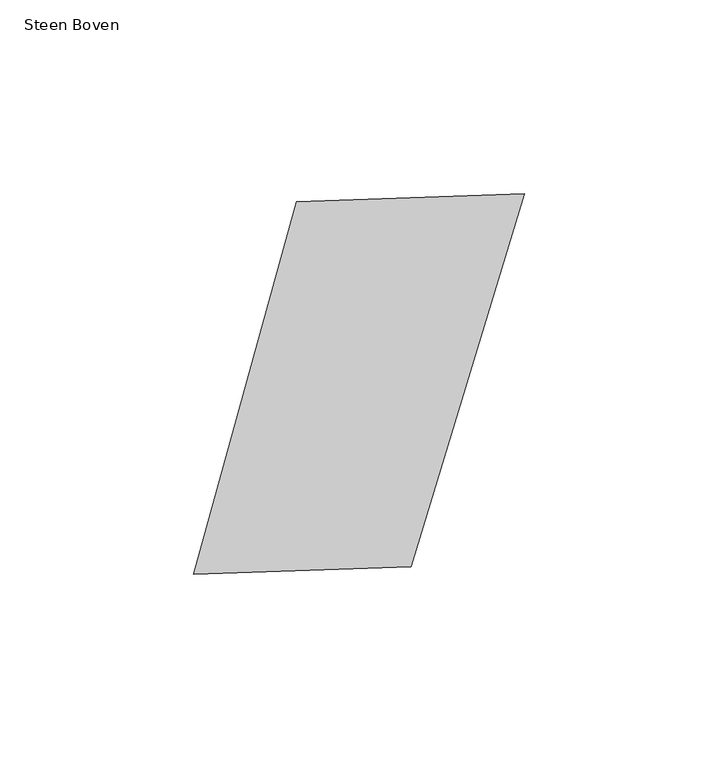
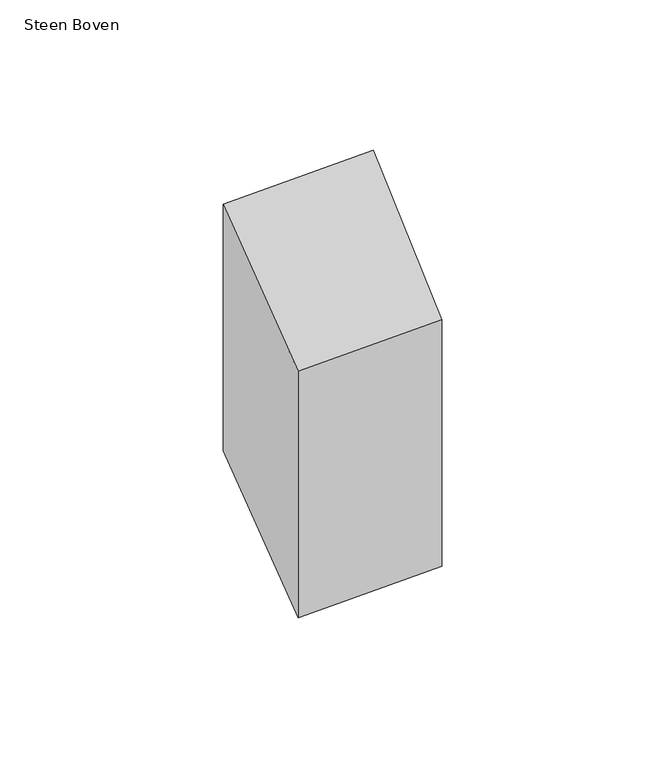
"""IFC4 building model written with IfcOpenShell, lengths in millimetres: proxy geometry, 00_GMA_steen_versie_4 : Steen Boven."""

from ifc_helpers import new_model, si_unit, origin, origin_with_axes, place, context, project, spatial, polyline, outline, extrude, source, transform, mapped, element, save


def steen_boven_ecc8bb5a(model_context):
    return source(origin(), model_context, "Body", "SweptSolid", [
        extrude(outline(polyline([(115.9629985, 119.0094516), (86.6063002, 22.6045748), (30.3176515, 20.5836998), (57.0367025, 116.8591339), (115.9629985, 119.0094516)])), origin_with_axes(), (0.0, 0.0, 1.0), 100.0),
    ])


if __name__ == "__main__":
    model = new_model("IFC4")
    model_context = context("Model", 3, world=origin())
    ifc_project = project(units=[si_unit("LENGTHUNIT", "METRE", prefix="MILLI")], contexts=[model_context])
    site = spatial("IfcSite", under=ifc_project)
    building = spatial("IfcBuilding", under=site)
    placement = place(None, origin())
    steen_boven_shape = steen_boven_ecc8bb5a(model_context)
    element("IfcBuildingElementProxy", 1, Name="00_GMA_steen_versie_4 : Steen Boven", ObjectType="00_GMA_steen_versie_4 : Steen Boven", at=placement, inside=building, context=model_context, shape_type="MappedRepresentation", body=[
        mapped(steen_boven_shape, transform((0.0, 0.0, 0.0), x_axis=(1.0, 0.0, 0.0), y_axis=(0.0, 1.0, 0.0), z_axis=(0.0, 0.0, 1.0))),
    ])
    save(model, "model.ifc")

# Revit data of these elements
# Type "00_GMA_steen_versie_4 : Steen Boven"
#   StootVoegHalfBoven [instance default] = 5 mm
#   StootVoegHalf [instance default] = 5 mm
#   StootVoegBreedteOnder = 10 mm
#   StootVoegBreedteBoven = 10 mm
#   Steendikte = 100 mm
#   LintVoegOnderHalf = 5 mm
#   LintVoegOnder = 10 mm
#   LintVoegBovenHalf = 0 mm
#   LintVoegBoven = 0 mm
#   materiaal = none
#   MateriaalVoeg = none
#   Default Elevation = 0
